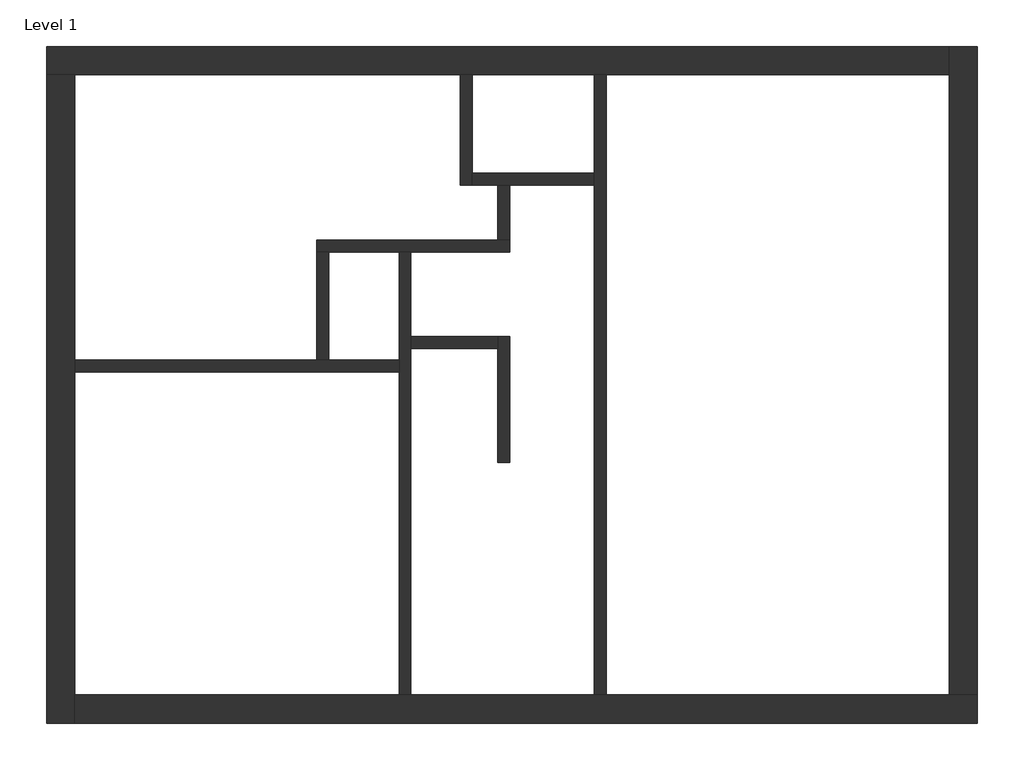
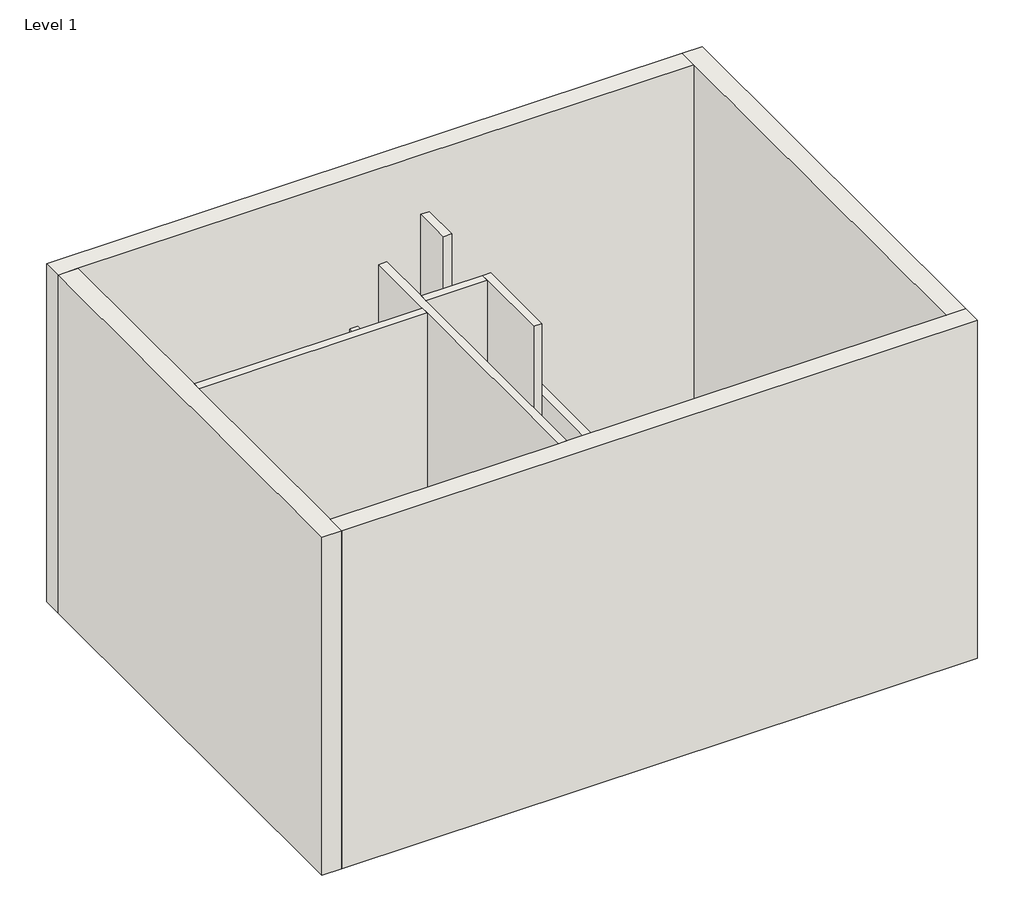
# One storey: 14 walls.
"""IFC4 building model written with IfcOpenShell, lengths in millimetres."""

from ifc_helpers import new_model, si_unit, origin, origin_with_axes, place, context, project, spatial, polyline, outline, extrude, faceted_brep, element, save

model = new_model("IFC4")

# Units and contexts
model_context = context("Model", 3, world=origin())
ifc_project = project(units=[si_unit("LENGTHUNIT", "METRE", prefix="MILLI")], contexts=[model_context])

# Site, building, storey
site = spatial("IfcSite", under=ifc_project)
building = spatial("IfcBuilding", under=site)
storey = spatial("IfcBuildingStorey", under=building, Name="Level 1", Elevation=0.0)

# Walls
placement = place(None, origin())
element("IfcWall", 1, ObjectType="Generic - 12\"", at=placement, inside=storey, context=model_context, shape_type="Brep", body=[
    faceted_brep([(-11569.7962638, 4537.786172, 0.0), (-11264.9962638, 4537.786172, 0.0), (-7099.3962638, 4537.786172, 0.0), (-6972.3962638, 4537.786172, 0.0), (-5651.5962638, 4537.786172, 0.0), (-5524.5962638, 4537.786172, 0.0), (-1816.1962638, 4537.786172, 0.0), (-1816.1962638, 4537.786172, 5486.4), (-11264.9962638, 4537.786172, 5486.4), (-11569.7962638, 4537.786172, 5486.4), (-11569.7962638, 4842.586172, 0.0), (-11569.7962638, 4842.586172, 5486.4), (-1816.1962638, 4842.586172, 5486.4), (-1816.1962638, 4842.586172, 0.0)], [[[0, 1, 2, 3, 4, 5, 6, 7, 8, 9]], [[10, 11, 12, 13]], [[6, 5, 4, 3, 2, 1, 0, 10, 13]], [[9, 8, 7, 12, 11]], [[0, 9, 11, 10]], [[7, 6, 13, 12]]]),
])
element("IfcWall", 2, ObjectType="Generic - 12\"", at=placement, inside=storey, context=model_context, shape_type="Brep", body=[
    faceted_brep([(-11264.9962638, -2472.613828, 0.0), (-11264.9962638, -2167.813828, 0.0), (-11264.9962638, 1324.686172, 0.0), (-11264.9962638, 1451.686172, 0.0), (-11264.9962638, 4537.786172, 0.0), (-11264.9962638, 4537.786172, 5486.4), (-11264.9962638, 1451.686172, 5486.4), (-11264.9962638, 1324.686172, 5486.4), (-11264.9962638, -2167.813828, 5486.4), (-11264.9962638, -2472.613828, 5486.4), (-11569.7962638, -2472.613828, 0.0), (-11569.7962638, -2472.613828, 5486.4), (-11569.7962638, 4537.786172, 5486.4), (-11569.7962638, 4537.786172, 0.0)], [[[0, 1, 2, 3, 4, 5, 6, 7, 8, 9]], [[10, 11, 12, 13]], [[4, 3, 2, 1, 0, 10, 13]], [[9, 8, 7, 6, 5, 12, 11]], [[0, 9, 11, 10]], [[5, 4, 13, 12]]]),
])
element("IfcWall", 3, ObjectType="Generic - 12\"", at=placement, inside=storey, context=model_context, shape_type="Brep", body=[
    faceted_brep([(-1511.3962638, -2167.813828, 0.0), (-1816.1962638, -2167.813828, 0.0), (-5524.5962638, -2167.813828, 0.0), (-5651.5962638, -2167.813828, 0.0), (-7632.7962638, -2167.813828, 0.0), (-7759.7962638, -2167.813828, 0.0), (-11264.9962638, -2167.813828, 0.0), (-11264.9962638, -2167.813828, 5486.4), (-7759.7962638, -2167.813828, 5486.4), (-7632.7962638, -2167.813828, 5486.4), (-1816.1962638, -2167.813828, 5486.4), (-1511.3962638, -2167.813828, 5486.4), (-1511.3962638, -2472.613828, 0.0), (-1511.3962638, -2472.613828, 5486.4), (-11264.9962638, -2472.613828, 5486.4), (-11264.9962638, -2472.613828, 0.0)], [[[0, 1, 2, 3, 4, 5, 6, 7, 8, 9, 10, 11]], [[12, 13, 14, 15]], [[6, 5, 4, 3, 2, 1, 0, 12, 15]], [[11, 10, 9, 8, 7, 14, 13]], [[0, 11, 13, 12]], [[7, 6, 15, 14]]]),
])
element("IfcWall", 4, ObjectType="Generic - 12\"", at=placement, inside=storey, context=model_context, shape_type="Brep", body=[
    faceted_brep([(-1816.1962638, 4842.586172, 0.0), (-1816.1962638, 4537.786172, 0.0), (-1816.1962638, -2167.813828, 0.0), (-1816.1962638, -2167.813828, 5486.4), (-1816.1962638, 4537.786172, 5486.4), (-1816.1962638, 4842.586172, 5486.4), (-1511.3962638, 4842.586172, 0.0), (-1511.3962638, 4842.586172, 5486.4), (-1511.3962638, -2167.813828, 5486.4), (-1511.3962638, -2167.813828, 0.0)], [[[0, 1, 2, 3, 4, 5]], [[6, 7, 8, 9]], [[2, 1, 0, 6, 9]], [[5, 4, 3, 8, 7]], [[0, 5, 7, 6]], [[3, 2, 9, 8]]]),
])
element("IfcWall", 5, ObjectType="Generic - 5\"", at=placement, inside=storey, context=model_context, shape_type="Brep", body=[
    faceted_brep([(-7632.7962638, -2167.813828, 0.0), (-7632.7962638, 1578.686172, 0.0), (-7632.7962638, 1705.686172, 0.0), (-7632.7962638, 2620.086172, 0.0), (-7632.7962638, 2620.086172, 5486.4), (-7632.7962638, 1705.686172, 5486.4), (-7632.7962638, 1578.686172, 5486.4), (-7632.7962638, -2167.813828, 5486.4), (-7759.7962638, -2167.813828, 0.0), (-7759.7962638, -2167.813828, 5486.4), (-7759.7962638, 1324.686172, 5486.4), (-7759.7962638, 1451.686172, 5486.4), (-7759.7962638, 2620.086172, 5486.4), (-7759.7962638, 2620.086172, 0.0), (-7759.7962638, 1451.686172, 0.0), (-7759.7962638, 1324.686172, 0.0)], [[[0, 1, 2, 3, 4, 5, 6, 7]], [[8, 9, 10, 11, 12, 13, 14, 15]], [[3, 2, 1, 0, 8, 15, 14, 13]], [[7, 6, 5, 4, 12, 11, 10, 9]], [[0, 7, 9, 8]], [[4, 3, 13, 12]]]),
])
element("IfcWall", 6, ObjectType="Generic - 5\"", at=placement, inside=storey, context=model_context, shape_type="SweptSolid", body=[
    extrude(outline(polyline([(-7632.7962638, 1705.686172), (-6692.9962638, 1705.686172), (-6692.9962638, 1578.686172), (-7632.7962638, 1578.686172), (-7632.7962638, 1705.686172)])), origin_with_axes(), (0.0, 0.0, 1.0), 5486.4),
])
element("IfcWall", 7, ObjectType="Generic - 5\"", at=placement, inside=storey, context=model_context, shape_type="Brep", body=[
    faceted_brep([(-8648.7962638, 2620.086172, 0.0), (-8521.7962638, 2620.086172, 0.0), (-7759.7962638, 2620.086172, 0.0), (-7632.7962638, 2620.086172, 0.0), (-6565.9962638, 2620.086172, 0.0), (-6565.9962638, 2620.086172, 3048.0), (-8521.7962638, 2620.086172, 3048.0), (-8648.7962638, 2620.086172, 3048.0), (-8648.7962638, 2747.086172, 0.0), (-8648.7962638, 2747.086172, 3048.0), (-6565.9962638, 2747.086172, 3048.0), (-6565.9962638, 2747.086172, 0.0), (-6692.9962638, 2747.086172, 0.0)], [[[0, 1, 2, 3, 4, 5, 6, 7]], [[8, 9, 10, 11, 12]], [[4, 3, 2, 1, 0, 8, 12, 11]], [[7, 6, 5, 10, 9]], [[0, 7, 9, 8]], [[5, 4, 11, 10]]]),
])
element("IfcWall", 8, ObjectType="Generic - 5\"", at=placement, inside=storey, context=model_context, shape_type="SweptSolid", body=[
    extrude(outline(polyline([(-8521.7962638, 2620.086172), (-8521.7962638, 1451.686172), (-8648.7962638, 1451.686172), (-8648.7962638, 2620.086172), (-8521.7962638, 2620.086172)])), origin_with_axes(), (0.0, 0.0, 1.0), 3048.0),
])
element("IfcWall", 9, ObjectType="Generic - 5\"", at=placement, inside=storey, context=model_context, shape_type="Brep", body=[
    faceted_brep([(-5651.5962638, 4537.786172, 0.0), (-5651.5962638, 3470.986172, 0.0), (-5651.5962638, 3343.986172, 0.0), (-5651.5962638, -2167.813828, 0.0), (-5651.5962638, -2167.813828, 3048.0), (-5651.5962638, 3343.986172, 3048.0), (-5651.5962638, 3470.986172, 3048.0), (-5651.5962638, 4537.786172, 3048.0), (-5524.5962638, 4537.786172, 0.0), (-5524.5962638, 4537.786172, 3048.0), (-5524.5962638, -2167.813828, 3048.0), (-5524.5962638, -2167.813828, 0.0)], [[[0, 1, 2, 3, 4, 5, 6, 7]], [[8, 9, 10, 11]], [[3, 2, 1, 0, 8, 11]], [[7, 6, 5, 4, 10, 9]], [[0, 7, 9, 8]], [[4, 3, 11, 10]]]),
])
element("IfcWall", 10, ObjectType="Generic - 5\"", at=placement, inside=storey, context=model_context, shape_type="Brep", body=[
    faceted_brep([(-7759.7962638, 1451.686172, 0.0), (-8521.7962638, 1451.686172, 0.0), (-8648.7962638, 1451.686172, 0.0), (-11264.9962638, 1451.686172, 0.0), (-11264.9962638, 1451.686172, 5486.4), (-7759.7962638, 1451.686172, 5486.4), (-7759.7962638, 1324.686172, 0.0), (-7759.7962638, 1324.686172, 5486.4), (-11264.9962638, 1324.686172, 5486.4), (-11264.9962638, 1324.686172, 0.0)], [[[0, 1, 2, 3, 4, 5]], [[6, 7, 8, 9]], [[3, 2, 1, 0, 6, 9]], [[5, 4, 8, 7]], [[4, 3, 9, 8]], [[0, 5, 7, 6]]]),
])
element("IfcWall", 11, ObjectType="Generic - 5\"", at=placement, inside=storey, context=model_context, shape_type="Brep", body=[
    faceted_brep([(-6565.9962638, 346.786172, 0.0), (-6565.9962638, 1705.686172, 0.0), (-6565.9962638, 1705.686172, 5486.4), (-6565.9962638, 346.786172, 5486.4), (-6692.9962638, 346.786172, 0.0), (-6692.9962638, 346.786172, 5486.4), (-6692.9962638, 1578.686172, 5486.4), (-6692.9962638, 1705.686172, 5486.4), (-6692.9962638, 1705.686172, 0.0), (-6692.9962638, 1578.686172, 0.0)], [[[0, 1, 2, 3]], [[4, 5, 6, 7, 8, 9]], [[1, 0, 4, 9, 8]], [[3, 2, 7, 6, 5]], [[0, 3, 5, 4]], [[2, 1, 8, 7]]]),
])
element("IfcWall", 12, ObjectType="Generic - 5\"", at=placement, inside=storey, context=model_context, shape_type="Brep", body=[
    faceted_brep([(-7099.3962638, 4537.786172, 0.0), (-7099.3962638, 3343.986172, 0.0), (-7099.3962638, 3343.986172, 3048.0), (-7099.3962638, 4537.786172, 3048.0), (-6972.3962638, 4537.786172, 0.0), (-6972.3962638, 4537.786172, 3048.0), (-6972.3962638, 3470.986172, 3048.0), (-6972.3962638, 3343.986172, 3048.0), (-6972.3962638, 3343.986172, 0.0), (-6972.3962638, 3470.986172, 0.0)], [[[0, 1, 2, 3]], [[4, 5, 6, 7, 8, 9]], [[1, 0, 4, 9, 8]], [[3, 2, 7, 6, 5]], [[0, 3, 5, 4]], [[2, 1, 8, 7]]]),
])
element("IfcWall", 13, ObjectType="Generic - 5\"", at=placement, inside=storey, context=model_context, shape_type="Brep", body=[
    faceted_brep([(-6972.3962638, 3343.986172, 0.0), (-6692.9962638, 3343.986172, 0.0), (-6565.9962638, 3343.986172, 0.0), (-5651.5962638, 3343.986172, 0.0), (-5651.5962638, 3343.986172, 3048.0), (-6972.3962638, 3343.986172, 3048.0), (-6972.3962638, 3470.986172, 0.0), (-6972.3962638, 3470.986172, 3048.0), (-5651.5962638, 3470.986172, 3048.0), (-5651.5962638, 3470.986172, 0.0)], [[[0, 1, 2, 3, 4, 5]], [[6, 7, 8, 9]], [[3, 2, 1, 0, 6, 9]], [[5, 4, 8, 7]], [[0, 5, 7, 6]], [[4, 3, 9, 8]]]),
])
element("IfcWall", 14, ObjectType="Generic - 5\"", at=placement, inside=storey, context=model_context, shape_type="Brep", body=[
    faceted_brep([(-6565.9962638, 2747.086172, 0.0), (-6565.9962638, 3343.986172, 0.0), (-6565.9962638, 3343.986172, 5486.4), (-6565.9962638, 2747.086172, 5486.4), (-6565.9962638, 2747.086172, 3048.0), (-6692.9962638, 2747.086172, 0.0), (-6692.9962638, 2747.086172, 5486.4), (-6692.9962638, 3343.986172, 5486.4), (-6692.9962638, 3343.986172, 0.0)], [[[0, 1, 2, 3, 4]], [[5, 6, 7, 8]], [[1, 0, 5, 8]], [[3, 2, 7, 6]], [[2, 1, 8, 7]], [[0, 4, 3, 6, 5]]]),
])

save(model, "model.ifc")

# Revit data of these elements
# Project information
#   Organization Name = "G3B Press"
#   Organization Description = "Paul F. Aubin Cosulting Services, Inc."
#   Building Name = "Revit Essentials for Architecture"
#   Author = "Paul F. Aubin"
#   Author Website = "https://www.paulaubin.com"
#   Copyright = "Copyright © 2020 Paul F Aubin, all rights reserved"
#   Project Issue Date = "8/1/2020"
#   Project Status = "Design Development"
#   Client Name = "Creating a Building Layout"
#   Project Address = "789 Main ST\nAnytown, IL 60000"
#   Project Name = "04 Residential-Walls"
#   Project Number = "2020.03A"
# Type "Generic - 12\""
#   Assembly Code = "B2010"
#   Layers, outside or top first: 1' - 0" no material (function 1)
# Type "Generic - 5\""
#   Assembly Code = "B2010"
#   Layers, outside or top first: 0' - 5" no material (function 1)
# Elements 1, 2, 3, 4 (IfcWall, "Generic - 12\"")
#   Top Offset = 0' - 0"
#   Base Offset = 0' - 0"
#   Unconnected Height = 18' - 0"
#   wall height = 18' - 0"
#   Phase Created = Existing
#   Base Constraint = Level 1
#   Materials on its faces: "Default Wall"
# Elements 5, 6, 10, 11, 14 (IfcWall, "Generic - 5\"")
#   Top Offset = 0' - 0"
#   Base Offset = 0' - 0"
#   Unconnected Height = 18' - 0"
#   wall height = 18' - 0"
#   Phase Created = Existing
#   Base Constraint = Level 1
#   Materials on its faces: "Default Wall"
# Elements 7, 8, 9, 12, 13 (IfcWall, "Generic - 5\"")
#   Top Offset = 0' - 0"
#   Base Offset = 0' - 0"
#   wall height = 10' - 0"
#   Phase Created = Existing
#   Base Constraint = Level 1
#   Top Constraint = Level 2
#   Materials on its faces: "Default Wall"
# Materials
#   "Default Wall": class "Miscellaneous", colour RGB 128 128 128, transparency 0, Cost = 0
